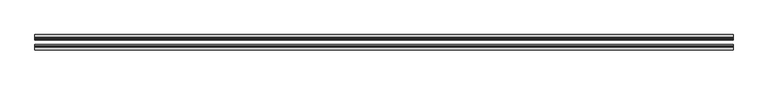
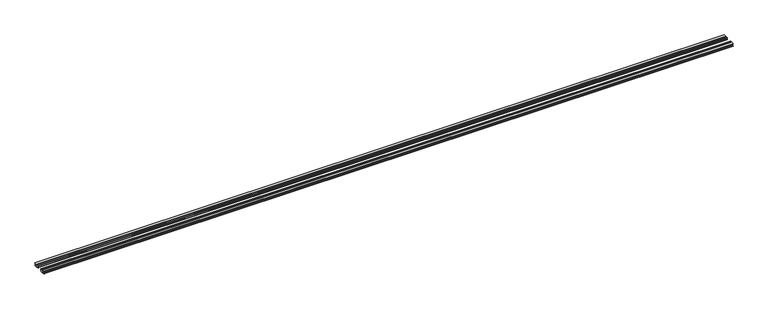
"""IFC4 building model written with IfcOpenShell, lengths in millimetres: proxy geometry, Generic Models 6:Generic Models 2:318829:Generic Models 2:318829 : Generic Models 6:Generic Models 2:318829:5 : Generic Models 6:Generic Models 2:318829:Generic Models 2:318829 : Generic Models 6:Generic Models 2:318829:300683."""

from ifc_helpers import new_model, si_unit, frame, origin, place, context, project, spatial, polyline, outline, extrude, source, transform, mapped, element, save


def generic_models_0e043b0c(model_context):
    return source(origin(), model_context, "Body", "SweptSolid", [
        extrude(outline(polyline([(-568227.2740999, 8555.9596728), (-568225.9836784, 8556.5391492), (-568224.0193157, 8558.1643773), (-568223.1187854, 8560.189749), (-568223.4229673, 8562.2984134), (-568224.8842748, 8564.1604896), (-568227.2740999, 8565.4846728), (-568218.4719617, 8565.4846728), (-568219.0380747, 8564.036028), (-568219.5086038, 8560.7221728), (-568219.0380747, 8557.4083176), (-568218.4719617, 8555.9596728), (-568227.2740999, 8555.9596728)])), frame((591391.6367242, 0.0, 0.0), z_axis=(1.0, 0.0, 0.0), x_axis=(0.0, 1.0, 0.0)), (0.0, 0.0, 1.0), 2438.4),
        extrude(outline(polyline([(-568232.4091752, 8556.0790786), (-568235.2735965, 8556.9987004), (-568237.2558376, 8558.6558015), (-568237.9632913, 8560.7221728), (-568237.2558376, 8562.7885441), (-568235.2735965, 8564.4456452), (-568232.4091752, 8565.365267), (-568230.8195413, 8565.4846728), (-568229.2299073, 8565.365267), (-568226.365486, 8564.4456452), (-568224.3832449, 8562.7885441), (-568223.6757913, 8560.7221728), (-568224.3832449, 8558.6558015), (-568226.365486, 8556.9987004), (-568229.2299073, 8556.0790786), (-568230.8195413, 8555.9596728), (-568232.4091752, 8556.0790786)])), frame((591391.6367242, 0.0, 0.0), z_axis=(1.0, 0.0, 0.0), x_axis=(0.0, 1.0, 0.0)), (0.0, 0.0, 1.0), 2438.4),
        extrude(outline(polyline([(-568263.5473576, 8555.9596728), (-568272.3494958, 8555.9596728), (-568271.7833829, 8557.4083176), (-568271.3128538, 8560.7221728), (-568271.7833829, 8564.036028), (-568272.3494958, 8565.4846728), (-568263.5473576, 8565.4846728), (-568265.9371827, 8564.1604896), (-568267.3984902, 8562.2984134), (-568267.7026721, 8560.189749), (-568266.8021418, 8558.1643773), (-568264.8377791, 8556.5391492), (-568263.5473576, 8555.9596728)])), frame((591391.6367242, 0.0, 0.0), z_axis=(1.0, 0.0, 0.0), x_axis=(0.0, 1.0, 0.0)), (0.0, 0.0, 1.0), 2438.4),
        extrude(outline(polyline([(-568258.4122823, 8556.0790786), (-568260.0019163, 8555.9596728), (-568261.5915502, 8556.0790786), (-568264.4559715, 8556.9987004), (-568266.4382126, 8558.6558015), (-568267.1456663, 8560.7221728), (-568266.4382126, 8562.7885441), (-568264.4559715, 8564.4456452), (-568261.5915502, 8565.365267), (-568260.0019163, 8565.4846728), (-568258.4122823, 8565.365267), (-568255.547861, 8564.4456452), (-568253.5656199, 8562.7885441), (-568252.8581663, 8560.7221728), (-568253.5656199, 8558.6558015), (-568255.547861, 8556.9987004), (-568258.4122823, 8556.0790786)])), frame((591391.6367242, 0.0, 0.0), z_axis=(1.0, 0.0, 0.0), x_axis=(0.0, 1.0, 0.0)), (0.0, 0.0, 1.0), 2438.4),
    ])


if __name__ == "__main__":
    model = new_model("IFC4")
    model_context = context("Model", 3, world=origin())
    ifc_project = project(units=[si_unit("LENGTHUNIT", "METRE", prefix="MILLI")], contexts=[model_context])
    site = spatial("IfcSite", under=ifc_project)
    building = spatial("IfcBuilding", under=site)
    placement = place(None, origin())
    generic_models_shape = generic_models_0e043b0c(model_context)
    element("IfcBuildingElementProxy", 1, Name="Generic Models 6:Generic Models 2:318829:Generic Models 2:318829 : Generic Models 6:Generic Models 2:318829:5 : Generic Models 6:Generic Models 2:318829:Generic Models 2:318829 : Generic Models 6:Generic Models 2:318829:300683", ObjectType="Generic Models 6:Generic Models 2:318829:Generic Models 2:318829 : Generic Models 6:Generic Models 2:318829:5 : Generic Models 6:Generic Models 2:318829:Generic Models 2:318829 : Generic Models 6:Generic Models 2:318829:300683", at=placement, inside=building, context=model_context, shape_type="MappedRepresentation", body=[
        mapped(generic_models_shape, transform((0.0, 0.0, 0.0), x_axis=(1.0, 0.0, 0.0), y_axis=(0.0, 1.0, 0.0), z_axis=(0.0, 0.0, 1.0))),
    ])
    save(model, "model.ifc")

# Revit data of these elements
# Type "Generic Models 6:Generic Models 2:318829:Generic Models 2:318829 : Generic Models 6:Generic Models 2:318829:5 : Generic Models 6:Generic Models 2:318829:Generic Models 2:318829 : Generic Models 6:Generic Models 2:318829:300683"
#   NameOverride = "Generic Models 6:Generic Models 2:318829:Generic Models 2:318829 : Generic Models 6:Generic Models 2:318829:300683"
#   ObjectTypeOverride = "Generic Models 2:318829 : Generic Models 6:Generic Models 2:318829"
#   Reference = "Generic Models 2"
#   Tag = "300683"
# Element 1 (IfcBuildingElementProxy, "Generic Models 6:Generic Models 2:318829:Generic Models 2:318829 : Generic Models 6:Generic Models 2:318829:5 : Generic Models 6:Generic Models 2:318829:Generic Models 2:318829 : Generic Models 6:Generic Models 2:318829:300683")
#   Materials on its faces: "SEALANT & BACKER ROD, IF NECESSARY"
# Materials
#   "SEALANT & BACKER ROD, IF NECESSARY": class "Unassigned", colour RGB 120 120 120, transparency 0, Cost = 0
